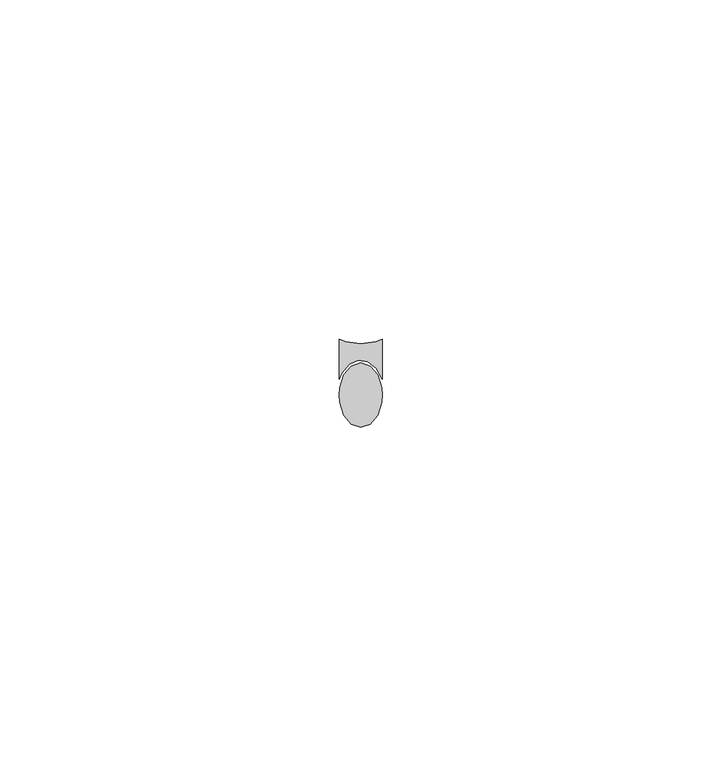
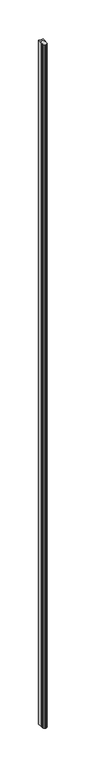
"""IFC4 building model written with IfcOpenShell, lengths in millimetres: proxy geometry, Generic Models 11:Generic Models 1:306267:Generic Models 1:306267 : Generic Models 11:Generic Models 1:306267:300405:Generic Models 1:306267:Generic Models 1:306267 : Generic Models 11:Generic Models 1:306267:300405 : Generic Models 11:Generic Models 1:306267:Generic Models 1:306267 : Generic Models 11:Generic Models 1:306267:300405:13 : Generic Models 11:Generic Models 1:306267:Generic Models 1:306267 : Generic Models 11:Generic Models 1:306267:300405:Generic Models 1:306267:Generic Models 1:306267 : Generic Models 11:Generic Models 1:306267:300405 : Generic Models 11:Generic Models 1:306267:Generic Models 1:306267 : Generic Models 11:Generic Models 1:306267:300405:300182."""

from ifc_helpers import new_model, si_unit, frame, origin, place, context, project, spatial, polyline, outline, extrude, source, transform, mapped, element, save


def generic_models_558b5538(model_context):
    return source(origin(), model_context, "Body", "SweptSolid", [
        extrude(outline(polyline([(593733.5341431, -557341.1942796), (593734.9117239, -557340.7226438), (593736.2893048, -557341.1942796), (593737.3940389, -557342.5157737), (593738.0071201, -557344.4253879), (593738.0867239, -557345.4851438), (593738.0071201, -557346.5448998), (593737.3940389, -557348.454514), (593736.2893048, -557349.7760081), (593734.9117239, -557350.2476438), (593733.5341431, -557349.7760081), (593732.429409, -557348.454514), (593731.8163278, -557346.5448998), (593731.7367239, -557345.4851438), (593731.8163278, -557344.4253879), (593732.429409, -557342.5157737), (593733.5341431, -557341.1942796)])), frame((0.0, 0.0, 5106.0759872), z_axis=(0.0, 0.0, 1.0), x_axis=(1.0, 0.0, 0.0)), (0.0, 0.0, 1.0), 1071.4379058),
        extrude(outline(polyline([(593737.1209607, -557337.6308328), (593738.0867239, -557337.2534241), (593738.0867239, -557343.1215163), (593737.2039351, -557341.5282995), (593735.962551, -557340.5540945), (593734.5567747, -557340.3513066), (593733.206527, -557340.9516601), (593732.1230415, -557342.2612353), (593731.7367239, -557343.1215163), (593731.7367239, -557337.2534241), (593732.7024872, -557337.6308328), (593734.9117239, -557337.9445188), (593737.1209607, -557337.6308328)])), frame((0.0, 0.0, 5106.0759872), z_axis=(0.0, 0.0, 1.0), x_axis=(1.0, 0.0, 0.0)), (0.0, 0.0, 1.0), 1071.4379058),
    ])


if __name__ == "__main__":
    model = new_model("IFC4")
    model_context = context("Model", 3, world=origin())
    ifc_project = project(units=[si_unit("LENGTHUNIT", "METRE", prefix="MILLI")], contexts=[model_context])
    site = spatial("IfcSite", under=ifc_project)
    building = spatial("IfcBuilding", under=site)
    placement = place(None, origin())
    generic_models_shape = generic_models_558b5538(model_context)
    element("IfcBuildingElementProxy", 1, Name="Generic Models 11:Generic Models 1:306267:Generic Models 1:306267 : Generic Models 11:Generic Models 1:306267:300405:Generic Models 1:306267:Generic Models 1:306267 : Generic Models 11:Generic Models 1:306267:300405 : Generic Models 11:Generic Models 1:306267:Generic Models 1:306267 : Generic Models 11:Generic Models 1:306267:300405:13 : Generic Models 11:Generic Models 1:306267:Generic Models 1:306267 : Generic Models 11:Generic Models 1:306267:300405:Generic Models 1:306267:Generic Models 1:306267 : Generic Models 11:Generic Models 1:306267:300405 : Generic Models 11:Generic Models 1:306267:Generic Models 1:306267 : Generic Models 11:Generic Models 1:306267:300405:300182", ObjectType="Generic Models 11:Generic Models 1:306267:Generic Models 1:306267 : Generic Models 11:Generic Models 1:306267:300405:Generic Models 1:306267:Generic Models 1:306267 : Generic Models 11:Generic Models 1:306267:300405 : Generic Models 11:Generic Models 1:306267:Generic Models 1:306267 : Generic Models 11:Generic Models 1:306267:300405:13 : Generic Models 11:Generic Models 1:306267:Generic Models 1:306267 : Generic Models 11:Generic Models 1:306267:300405:Generic Models 1:306267:Generic Models 1:306267 : Generic Models 11:Generic Models 1:306267:300405 : Generic Models 11:Generic Models 1:306267:Generic Models 1:306267 : Generic Models 11:Generic Models 1:306267:300405:300182", at=placement, inside=building, context=model_context, shape_type="MappedRepresentation", body=[
        mapped(generic_models_shape, transform((0.0, 0.0, 0.0), x_axis=(1.0, 0.0, 0.0), y_axis=(0.0, 1.0, 0.0), z_axis=(0.0, 0.0, 1.0))),
    ])
    save(model, "model.ifc")

# Revit data of these elements
# Type "Generic Models 11:Generic Models 1:306267:Generic Models 1:306267 : Generic Models 11:Generic Models 1:306267:300405:Generic Models 1:306267:Generic Models 1:306267 : Generic Models 11:Generic Models 1:306267:300405 : Generic Models 11:Generic Models 1:306267:Generic Models 1:306267 : Generic Models 11:Generic Models 1:306267:300405:13 : Generic Models 11:Generic Models 1:306267:Generic Models 1:306267 : Generic Models 11:Generic Models 1:306267:300405:Generic Models 1:306267:Generic Models 1:306267 : Generic Models 11:Generic Models 1:306267:300405 : Generic Models 11:Generic Models 1:306267:Generic Models 1:306267 : Generic Models 11:Generic Models 1:306267:300405:300182"
#   NameOverride = "Generic Models 11:Generic Models 1:306267:Generic Models 1:306267 : Generic Models 11:Generic Models 1:306267:300405:Generic Models 1:306267:Generic Models 1:306267 : Generic Models 11:Generic Models 1:306267:300405 : Generic Models 11:Generic Models 1:306267:Generic Models 1:306267 : Generic Models 11:Generic Models 1:306267:300405:300182"
#   ObjectTypeOverride = "Generic Models 1:306267:Generic Models 1:306267 : Generic Models 11:Generic Models 1:306267:300405 : Generic Models 11:Generic Models 1:306267:Generic Models 1:306267 : Generic Models 11:Generic Models 1:306267:300405"
#   Reference = "Generic Models 1"
#   Tag = "300182"
# Element 1 (IfcBuildingElementProxy, "Generic Models 11:Generic Models 1:306267:Generic Models 1:306267 : Generic Models 11:Generic Models 1:306267:300405:Generic Models 1:306267:Generic Models 1:306267 : Generic Models 11:Generic Models 1:306267:300405 : Generic Models 11:Generic Models 1:306267:Generic Models 1:306267 : Generic Models 11:Generic Models 1:306267:300405:13 : Generic Models 11:Generic Models 1:306267:Generic Models 1:306267 : Generic Models 11:Generic Models 1:306267:300405:Generic Models 1:306267:Generic Models 1:306267 : Generic Models 11:Generic Models 1:306267:300405 : Generic Models 11:Generic Models 1:306267:Generic Models 1:306267 : Generic Models 11:Generic Models 1:306267:300405:300182")
#   Materials on its faces: "SEALANT & BACKER ROD, IF NECESSARY"
# Materials
#   "SEALANT & BACKER ROD, IF NECESSARY": class "Unassigned", colour RGB 120 120 120, transparency 0, Cost = 0
